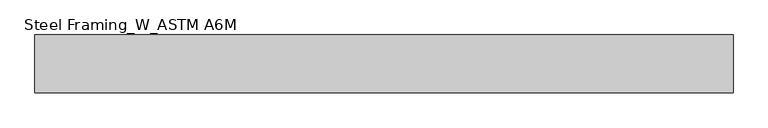
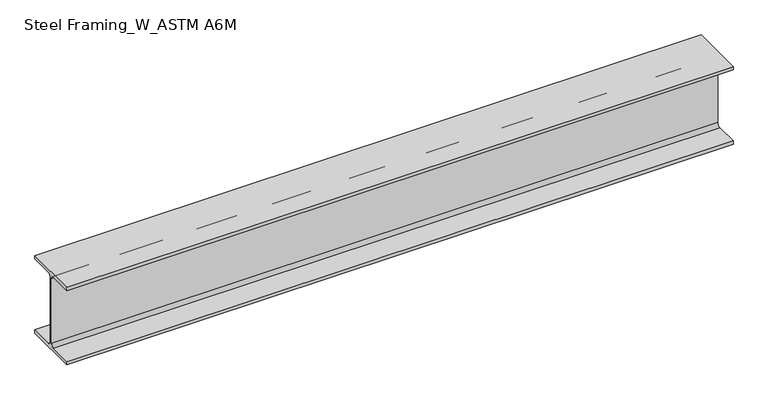
"""IFC4 building model written with IfcOpenShell, lengths in millimetres: beam geometry, Steel Framing_W_ASTM A6M : H_SB_AR_S02_W310x60_B5."""

from ifc_helpers import new_model, si_unit, point, frame, frame_2d, origin, place, context, project, spatial, polyline, circle_curve, trimmed, segment, composite_curve, outline, extrude, source, transform, mapped, element, save


def steel_framing_w_astm_a6m_8815720a(model_context):
    return source(origin(), model_context, "Body", "SweptSolid", [
        extrude(outline(composite_curve([segment(polyline([(101.5, -137.9), (101.5, -151.0), (-101.5, -151.0), (-101.5, -137.9), (-16.545, -137.9)]), True, "CONTINUOUS"), segment(trimmed(circle_curve(frame_2d((-16.545, -125.1)), 12.8), [point((-16.545, -137.9))], [point((-3.745, -125.1))], True, "CARTESIAN"), True, "CONTINUOUS"), segment(polyline([(-3.745, -125.1), (-3.745, 125.1)]), True, "CONTINUOUS"), segment(trimmed(circle_curve(frame_2d((-16.545, 125.1)), 12.8), [point((-3.745, 125.1))], [point((-16.545, 137.9))], True, "CARTESIAN"), True, "CONTINUOUS"), segment(polyline([(-16.545, 137.9), (-101.5, 137.9), (-101.5, 151.0), (101.5, 151.0), (101.5, 137.9), (16.545, 137.9)]), True, "CONTINUOUS"), segment(trimmed(circle_curve(frame_2d((16.545, 125.1)), 12.8), [point((16.545, 137.9))], [point((3.745, 125.1))], True, "CARTESIAN"), True, "CONTINUOUS"), segment(polyline([(3.745, 125.1), (3.745, -125.1)]), True, "CONTINUOUS"), segment(trimmed(circle_curve(frame_2d((16.545, -125.1)), 12.8), [point((3.745, -125.1))], [point((16.545, -137.9))], True, "CARTESIAN"), True, "CONTINUOUS"), segment(polyline([(16.545, -137.9), (101.5, -137.9)]), True, "CONTINUOUS")], self_intersect=False)), frame((-1096.3, 0.0, 0.0), z_axis=(1.0, 0.0, 0.0), x_axis=(0.0, 1.0, 0.0)), (0.0, 0.0, 1.0), 2447.8),
    ])


if __name__ == "__main__":
    model = new_model("IFC4")
    model_context = context("Model", 3, world=origin())
    ifc_project = project(units=[si_unit("LENGTHUNIT", "METRE", prefix="MILLI")], contexts=[model_context])
    site = spatial("IfcSite", under=ifc_project)
    building = spatial("IfcBuilding", under=site)
    placement = place(None, origin())
    steel_framing_w_astm_a6m_shape = steel_framing_w_astm_a6m_8815720a(model_context)
    element("IfcBeam", 1, ObjectType="Steel Framing_W_ASTM A6M : H_SB_AR_S02_W310x60_B5", at=placement, inside=building, context=model_context, shape_type="MappedRepresentation", body=[
        mapped(steel_framing_w_astm_a6m_shape, transform((0.0, 0.0, 0.0), x_axis=(1.0, 0.0, 0.0), y_axis=(0.0, 1.0, 0.0), z_axis=(0.0, 0.0, 1.0))),
    ])
    save(model, "model.ifc")

# Revit data of these elements
# Type "Steel Framing_W_ASTM A6M : H_SB_AR_S02_W310x60_B5"
#   Type Mark = "B5"
#   Section Name Key = "W12x40"
#   Width = 20.3 cm
#   Web Thickness = 0.749 cm
#   Web Fillet = 1.28 cm
#   Warping Constant = 387000.0 cm⁶
#   Torsional Moment of Inertia = 37.70 cm⁴
#   Section Area = 75.5 cm²
#   Plastic Modulus weak axis = 275.0 cm³
#   Plastic Modulus strong axis = 934.0 cm³
#   Perimeter = 1.38 m²/m
#   Nominal Weight = 60.00 kgf/m
#   Moment of Inertia weak axis = 1840.00 cm⁴
#   Moment of Inertia strong axis = 12800.00 cm⁴
#   Height = 30.2 cm
#   Flange Thickness = 1.31 cm
#   Elastic Modulus weak axis = 180.0 cm³
#   Elastic Modulus strong axis = 844.0 cm³
#   Centroid Vertical = 15.1 cm
#   Centroid Horizontal = 10.15 cm
#   Length [instance default] = 1500 mm
#   Structural Material [instance default] = Steel, 45-345
#   Bolt Spacing = 0
#   Assembly Code = ""
# Element 1 (IfcBeam, "Steel Framing_W_ASTM A6M : H_SB_AR_S02_W310x60_B5")
#   Materials on its faces: "Steel, 45-345"
# Materials
#   "Steel, 45-345": class "Metal", colour RGB 189 187 185, transparency 0, Description = "Steel 345 MPa", Cost = 0
